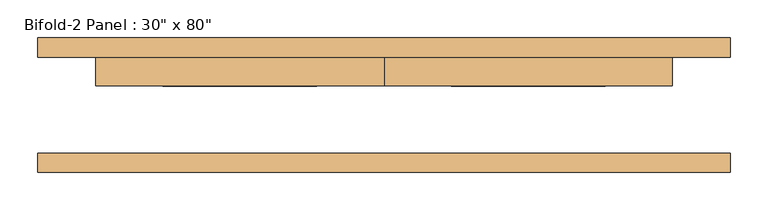
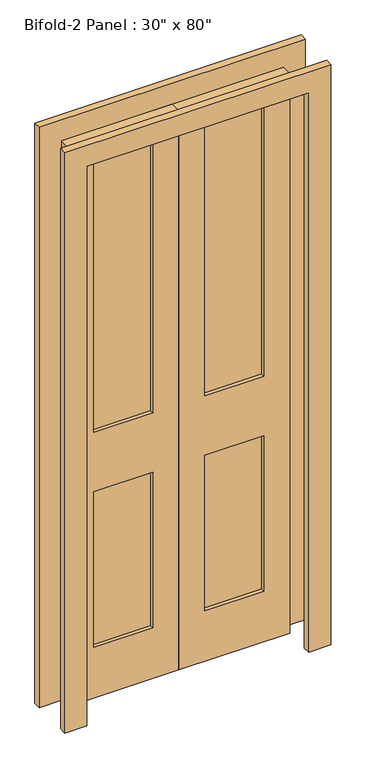
"""IFC4 building model written with IfcOpenShell, lengths in millimetres: door geometry."""

from ifc_helpers import new_model, si_unit, frame, origin, place, context, project, spatial, polyline, outline, extrude, source, transform, mapped, element, save


def door_1a011cc6(model_context):
    return source(origin(), model_context, "Body", "SweptSolid", [
        extrude(outline(polyline([(2032.0, 0.0), (2032.0, -381.0), (0.0, -381.0), (0.0, 0.0), (2032.0, 0.0)]), holes=[polyline([(1943.1, -88.9), (965.11872, -88.9), (965.11872, -292.1), (1943.1, -292.1), (1943.1, -88.9)]), polyline([(749.3, -88.9), (184.15, -88.9), (184.15, -292.1), (749.3, -292.1), (749.3, -88.9)])]), frame((0.0, 25.4, 0.0), z_axis=(0.0, 1.0, 0.0), x_axis=(0.0, 0.0, 1.0)), (0.0, 0.0, 1.0), 38.1),
        extrude(outline(polyline([(-88.9, 38.1), (-292.1, 38.1), (-292.1, 50.8), (-88.9, 50.8), (-88.9, 38.1)])), frame((0.0, 0.0, 965.11872), z_axis=(0.0, 0.0, 1.0), x_axis=(1.0, 0.0, 0.0)), (0.0, 0.0, 1.0), 977.98128),
        extrude(outline(polyline([(-88.9, 38.1), (-292.1, 38.1), (-292.1, 50.8), (-88.9, 50.8), (-88.9, 38.1)])), frame((0.0, 0.0, 184.15), z_axis=(0.0, 0.0, 1.0), x_axis=(1.0, 0.0, 0.0)), (0.0, 0.0, 1.0), 565.15),
        extrude(outline(polyline([(292.1, 38.1), (88.9, 38.1), (88.9, 50.8), (292.1, 50.8), (292.1, 38.1)])), frame((0.0, 0.0, 965.11872), z_axis=(0.0, 0.0, 1.0), x_axis=(1.0, 0.0, 0.0)), (0.0, 0.0, 1.0), 977.98128),
        extrude(outline(polyline([(292.1, 38.1), (88.9, 38.1), (88.9, 50.8), (292.1, 50.8), (292.1, 38.1)])), frame((0.0, 0.0, 184.15), z_axis=(0.0, 0.0, 1.0), x_axis=(1.0, 0.0, 0.0)), (0.0, 0.0, 1.0), 565.15),
        extrude(outline(polyline([(2108.2, -457.2), (0.0, -457.2), (0.0, -381.0), (2032.0, -381.0), (2032.0, 381.0), (0.0, 381.0), (0.0, 457.2), (2108.2, 457.2), (2108.2, -457.2)])), frame((0.0, 63.5, 0.0), z_axis=(0.0, 1.0, 0.0), x_axis=(0.0, 0.0, 1.0)), (0.0, 0.0, 1.0), 25.4),
        extrude(outline(polyline([(2108.2, 457.2), (2108.2, -457.2), (0.0, -457.2), (0.0, -381.0), (2032.0, -381.0), (2032.0, 381.0), (0.0, 381.0), (0.0, 457.2), (2108.2, 457.2)])), frame((0.0, -88.9, 0.0), z_axis=(0.0, 1.0, 0.0), x_axis=(0.0, 0.0, 1.0)), (0.0, 0.0, 1.0), 25.4),
        extrude(outline(polyline([(2032.0, 381.0), (2032.0, 0.0), (0.0, 0.0), (0.0, 381.0), (2032.0, 381.0)]), holes=[polyline([(1943.1, 88.9), (1943.1, 292.1), (965.11872, 292.1), (965.11872, 88.9), (1943.1, 88.9)]), polyline([(749.3, 88.9), (749.3, 292.1), (184.15, 292.1), (184.15, 88.9), (749.3, 88.9)])]), frame((0.0, 25.4, 0.0), z_axis=(0.0, 1.0, 0.0), x_axis=(0.0, 0.0, 1.0)), (0.0, 0.0, 1.0), 38.1),
    ])


if __name__ == "__main__":
    model = new_model("IFC4")
    model_context = context("Model", 3, world=origin())
    ifc_project = project(units=[si_unit("LENGTHUNIT", "METRE", prefix="MILLI")], contexts=[model_context])
    site = spatial("IfcSite", under=ifc_project)
    building = spatial("IfcBuilding", under=site)
    placement = place(None, origin())
    door_shape = door_1a011cc6(model_context)
    element("IfcDoor", 1, ObjectType="Bifold-2 Panel : 30\" x 80\"", at=placement, inside=building, context=model_context, shape_type="MappedRepresentation", body=[
        mapped(door_shape, transform((0.0, 0.0, 0.0), x_axis=(1.0, 0.0, 0.0), y_axis=(0.0, 1.0, 0.0), z_axis=(0.0, 0.0, 1.0))),
    ])
    save(model, "model.ifc")

# Revit data of these elements
# Type "Bifold-2 Panel : 30\" x 80\""
#   Type Mark = "11"
#   Construction Type Id = "MDOOR"
#   Assembly Code = "C1020"
#   Analytic Construction = "Metal"
#   Thickness = 0' - 1 1/2"
#   Thermal Resistance (R) = 1.5338 (h·ft²·°F)/BTU
#   Heat Transfer Coefficient (U) = 0.651978 BTU/(h·ft²·°F)
#   Height = 6' - 8"
#   Trim Projection Ext = 0' - 1"
#   Trim Projection Int = 0' - 1"
#   Trim Width = 0' - 3"
#   Width = 2' - 6"
#   Define Thermal Properties by = 1
#   Door Material = Door - Panel
#   Frame Material = Door - Frame
#   Visual Light Transmittance = 0
#   Solar Heat Gain Coefficient = 0
#   Function = (empty or 0)
#   Wall Closure = (empty or 0)
# Element 1 (IfcDoor, "Bifold-2 Panel : 30\" x 80\"")
#   Materials on its faces: "Door - Panel", "Door - Frame"
# Materials
#   "Door - Panel": class "Wood", colour RGB 210 159 95, transparency 0, Cost = 0
#   "Door - Frame": class "Miscellaneous", colour RGB 118 70 51, transparency 0, Cost = 0
